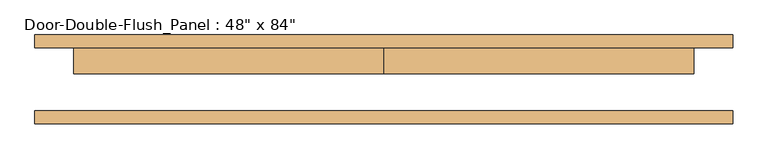
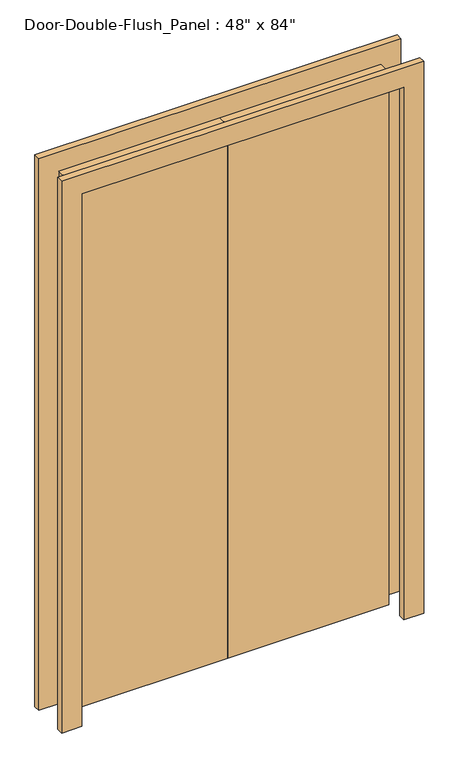
"""IFC4 building model written with IfcOpenShell, lengths in millimetres: door geometry."""

import ifcopenshell
import ifcopenshell.guid

model = None  # the IFC model being written
_history = None  # IfcOwnerHistory: only IFC2X3 demands one
_inside = {}  # id of a spatial element -> (the spatial element, [elements in it])
_under = {}  # id of a project, library or spatial element -> (it, [spatial elements below it])
_declared = {}  # id of a project -> (the project, [libraries it declares])
_typed = {}  # id of a type object -> (the type object, [elements of that type])
_made_of = {}  # id of a material, layer set ... -> (it, [elements and type objects made of it])


def new_model(schema):
    """Start an empty IFC model of exactly this schema.

    Asked for "IFC4X3", IfcOpenShell would pick the latest addendum, in which some entities
    have other attributes; the version numbers below select the first issue.
    IFC2X3 requires an IfcOwnerHistory on every rooted entity: one is made here for all.
    """
    global model, _history
    if schema == "IFC4X3":
        model = ifcopenshell.file(schema_version=(4, 3, 0, 0))
    else:
        model = ifcopenshell.file(schema=schema)
    _inside.clear()
    _under.clear()
    _declared.clear()
    _typed.clear()
    _made_of.clear()
    _history = None
    if model.schema == "IFC2X3":
        org = make("IfcOrganization", Name="unknown")
        user = make(
            "IfcPersonAndOrganization",
            ThePerson=make("IfcPerson", FamilyName="unknown"),
            TheOrganization=org,
        )
        app = make(
            "IfcApplication",
            ApplicationDeveloper=org,
            Version="unknown",
            ApplicationFullName="unknown",
            ApplicationIdentifier="unknown",
        )
        _history = make(
            "IfcOwnerHistory",
            OwningUser=user,
            OwningApplication=app,
            ChangeAction="ADDED",
            CreationDate=0,
        )
    return model


def make(cls, **values):
    """One entity of the class cls with the attributes given. An attribute that is None is left unset."""
    return model.create_entity(
        cls, **{name: value for name, value in values.items() if value is not None}
    )


def rooted(cls, **values):
    """An entity with a GlobalId (a new one), such as an element, a storey or a relation."""
    return make(cls, GlobalId=ifcopenshell.guid.new(), OwnerHistory=_history, **values)


def si_unit(unit_type, name, prefix=None):
    """IfcSIUnit, for example si_unit("LENGTHUNIT", "METRE", prefix="MILLI")."""
    return make("IfcSIUnit", UnitType=unit_type, Prefix=prefix, Name=name)


def assignment(units):
    """IfcUnitAssignment: the units of a project."""
    return None if units is None else make("IfcUnitAssignment", Units=units)


def point(xyz):
    """IfcCartesianPoint."""
    return None if xyz is None else make("IfcCartesianPoint", Coordinates=xyz)


def direction(xyz):
    """IfcDirection."""
    return None if xyz is None else make("IfcDirection", DirectionRatios=xyz)


def frame(location, z_axis=None, x_axis=None):
    """IfcAxis2Placement3D, a coordinate frame: its origin and axes. An axis left out is left unset."""
    return make(
        "IfcAxis2Placement3D",
        Location=point(location),
        Axis=direction(z_axis),
        RefDirection=direction(x_axis),
    )


def origin():
    """The frame at (0, 0, 0) with its axes left unset."""
    return frame((0.0, 0.0, 0.0))


def origin_with_axes():
    """The frame at (0, 0, 0) with the z axis (0, 0, 1) and the x axis (1, 0, 0) written out."""
    return frame((0.0, 0.0, 0.0), z_axis=(0.0, 0.0, 1.0), x_axis=(1.0, 0.0, 0.0))


def place(relative_to, where):
    """IfcLocalPlacement: puts the frame where relative to a parent placement (None: the world)."""
    return make(
        "IfcLocalPlacement", PlacementRelTo=relative_to, RelativePlacement=where
    )


def context(
    kind, dimensions, precision=None, world=None, true_north=None, identifier=None
):
    """IfcGeometricRepresentationContext, for example the 3D "Model" context."""
    return make(
        "IfcGeometricRepresentationContext",
        ContextIdentifier=identifier,
        ContextType=kind,
        CoordinateSpaceDimension=dimensions,
        Precision=precision,
        WorldCoordinateSystem=world,
        TrueNorth=true_north,
    )


def project(units=None, contexts=None):
    """IfcProject with its units and contexts."""
    return rooted(
        "IfcProject",
        Name="project",
        RepresentationContexts=contexts,
        UnitsInContext=assignment(units),
    )


def spatial(cls, under=None, at=None, **own):
    """A site, building, storey or space (cls), placed at a placement, below another one or the project."""
    s = rooted(cls, ObjectPlacement=at, **own)
    if under is not None:
        _under.setdefault(under.id(), (under, []))[1].append(s)
    return s


def polyline(points):
    """IfcPolyline through the points."""
    return make("IfcPolyline", Points=[point(p) for p in points])


def outline(outer, holes=None, kind="AREA"):
    """IfcArbitraryClosedProfileDef: a profile drawn as a closed curve; with holes, ...WithVoids."""
    if holes is None:
        return make("IfcArbitraryClosedProfileDef", ProfileType=kind, OuterCurve=outer)
    return make(
        "IfcArbitraryProfileDefWithVoids",
        ProfileType=kind,
        OuterCurve=outer,
        InnerCurves=holes,
    )


def extrude(swept, where, along, depth):
    """IfcExtrudedAreaSolid: the profile swept, set in the frame where, extruded along a direction by depth."""
    return make(
        "IfcExtrudedAreaSolid",
        SweptArea=swept,
        Position=where,
        ExtrudedDirection=direction(along),
        Depth=depth,
    )


def shape(context_of_items, identifier, shape_type, items):
    """IfcShapeRepresentation: the items that make up one representation, for example the "Body"."""
    return make(
        "IfcShapeRepresentation",
        ContextOfItems=context_of_items,
        RepresentationIdentifier=identifier,
        RepresentationType=shape_type,
        Items=items,
    )


def source(mapping_origin, context_of_items, identifier, shape_type, items):
    """IfcRepresentationMap: a shape defined once, which mapped items show again and again."""
    return make(
        "IfcRepresentationMap",
        MappingOrigin=mapping_origin,
        MappedRepresentation=shape(context_of_items, identifier, shape_type, items),
    )


def transform(
    local_origin,
    x_axis=None,
    y_axis=None,
    z_axis=None,
    scale=None,
    scale2=None,
    scale3=None,
    uniform=True,
):
    """IfcCartesianTransformationOperator3D, or its non-uniform kind. x_axis, y_axis, z_axis: its Axis1, 2, 3."""
    if uniform:
        return make(
            "IfcCartesianTransformationOperator3D",
            Axis1=direction(x_axis),
            Axis2=direction(y_axis),
            LocalOrigin=point(local_origin),
            Scale=scale,
            Axis3=direction(z_axis),
        )
    return make(
        "IfcCartesianTransformationOperator3DnonUniform",
        Axis1=direction(x_axis),
        Axis2=direction(y_axis),
        LocalOrigin=point(local_origin),
        Scale=scale,
        Axis3=direction(z_axis),
        Scale2=scale2,
        Scale3=scale3,
    )


def mapped(mapping_source, mapping_target):
    """IfcMappedItem: shows the shape of a source again, moved by a transform."""
    return make(
        "IfcMappedItem", MappingSource=mapping_source, MappingTarget=mapping_target
    )


def made_of(thing, what):
    """Note that an element or type object is made of a material, layer set ...; save() writes the relation."""
    if what is not None:
        _made_of.setdefault(what.id(), (what, []))[1].append(thing)
    return thing


def element(
    cls,
    number,
    at=None,
    inside=None,
    cuts=None,
    type_object=None,
    material=None,
    context=None,
    identifier="Body",
    shape_type=None,
    held_by="IfcProductDefinitionShape",
    body=None,
    shapes=None,
    **own,
):
    """One element of the class cls, such as IfcWall. Its Tag is "e" and its number.

    at: its placement. inside: the storey or other place that contains it. cuts: it is an
    opening in that element (IfcRelVoidsElement). A single representation is given by context,
    identifier, shape_type and body (its items); several are given by shapes. held_by: the class
    of the entity that holds the representations. save() writes the other relations.
    """
    e = rooted(cls, Tag="e%d" % number, ObjectPlacement=at, **own)
    if body is not None:
        shapes = [shape(context, identifier, shape_type, body)]
    if shapes is not None:
        e.Representation = make(held_by, Representations=shapes)
    if inside is not None:
        _inside.setdefault(inside.id(), (inside, []))[1].append(e)
    if cuts is not None:
        rooted(
            "IfcRelVoidsElement", RelatingBuildingElement=cuts, RelatedOpeningElement=e
        )
    if type_object is not None:
        _typed.setdefault(type_object.id(), (type_object, []))[1].append(e)
    return made_of(e, material)


def aggregate(whole, parts):
    """IfcRelAggregates: a whole, such as a stair, and the parts it consists of."""
    return rooted("IfcRelAggregates", RelatingObject=whole, RelatedObjects=parts)


def save(model, path):
    """Write the relations noted so far, then the file.

    IfcRelAggregates (storeys below a building ...), IfcRelContainedInSpatialStructure (elements
    in a storey), IfcRelDefinesByType, IfcRelAssociatesMaterial and IfcRelDeclares: one each for
    every whole, place, type object, material and project.
    """
    for whole, parts in _under.values():
        aggregate(whole, parts)
    for where, things in _inside.values():
        rooted(
            "IfcRelContainedInSpatialStructure",
            RelatedElements=things,
            RelatingStructure=where,
        )
    for kind, things in _typed.values():
        rooted("IfcRelDefinesByType", RelatedObjects=things, RelatingType=kind)
    for what, things in _made_of.values():
        rooted("IfcRelAssociatesMaterial", RelatedObjects=things, RelatingMaterial=what)
    for by, libraries in _declared.values():
        rooted("IfcRelDeclares", RelatingContext=by, RelatedDefinitions=libraries)
    model.write(path)


def door_4331e645(model_context):
    return source(origin(), model_context, "Body", "SweptSolid", [
        extrude(outline(polyline([(2133.6, -609.6), (2133.6, 609.6), (0.0, 609.6), (0.0, 685.8), (2209.8, 685.8), (2209.8, -685.8), (0.0, -685.8), (0.0, -609.6), (2133.6, -609.6)])), frame((0.0, -87.3125, 0.0), z_axis=(0.0, 1.0, 0.0), x_axis=(0.0, 0.0, 1.0)), (0.0, 0.0, 1.0), 25.4),
        extrude(outline(polyline([(2133.6, -609.6), (2133.6, 609.6), (0.0, 609.6), (0.0, 685.8), (2209.8, 685.8), (2209.8, -685.8), (0.0, -685.8), (0.0, -609.6), (2133.6, -609.6)])), frame((0.0, 61.9125, 0.0), z_axis=(0.0, 1.0, 0.0), x_axis=(0.0, 0.0, 1.0)), (0.0, 0.0, 1.0), 25.4),
        extrude(outline(polyline([(0.0, 61.9125), (609.6, 61.9125), (609.6, 11.1125), (0.0, 11.1125), (0.0, 61.9125)])), origin_with_axes(), (0.0, 0.0, 1.0), 2133.6),
        extrude(outline(polyline([(-609.6, 61.9125), (0.0, 61.9125), (0.0, 11.1125), (-609.6, 11.1125), (-609.6, 61.9125)])), origin_with_axes(), (0.0, 0.0, 1.0), 2133.6),
    ])


if __name__ == "__main__":
    model = new_model("IFC4")
    model_context = context("Model", 3, world=origin())
    ifc_project = project(units=[si_unit("LENGTHUNIT", "METRE", prefix="MILLI")], contexts=[model_context])
    site = spatial("IfcSite", under=ifc_project)
    building = spatial("IfcBuilding", under=site)
    placement = place(None, origin())
    door_shape = door_4331e645(model_context)
    element("IfcDoor", 1, ObjectType="Door-Double-Flush_Panel : 48\" x 84\"", at=placement, inside=building, context=model_context, shape_type="MappedRepresentation", body=[
        mapped(door_shape, transform((0.0, 0.0, 0.0), x_axis=(1.0, 0.0, 0.0), y_axis=(0.0, 1.0, 0.0), z_axis=(0.0, 0.0, 1.0))),
    ])
    save(model, "model.ifc")

# Revit data of these elements
# Type "Door-Double-Flush_Panel : 48\" x 84\""
#   Type Mark = "8"
#   Fire Rating = "60 Mins"
#   Construction Type Id = "DOOR"
#   Assembly Code = "C1020"
#   Analytic Construction = "Wooden"
#   Thickness = 0' - 2"
#   Thermal Resistance (R) = 2.5876 (h·ft²·°F)/BTU
#   Swing Angle [instance default] = 90.00°
#   Panel Width = 2' - 0"
#   Heat Transfer Coefficient (U) = 0.3865 BTU/(h·ft²·°F)
#   Height = 7' - 0"
#   Trim Projection Ext = 0' - 1"
#   Trim Projection Int = 0' - 1"
#   Trim Width = 0' - 3"
#   Width = 4' - 0"
#   Define Thermal Properties by = 1
#   Panel Material = Wood - Birch - Solid Stained Light Low Gloss
#   Trim Material = Paint - Sienna
#   Visual Light Transmittance = 0
#   Solar Heat Gain Coefficient = 0
#   Function = (empty or 0)
#   Wall Closure = (empty or 0)
# Element 1 (IfcDoor, "Door-Double-Flush_Panel : 48\" x 84\"")
#   Materials on its faces: "Paint - Sienna", "Wood - Birch - Solid Stained Light Low Gloss"
# Materials
#   "Wood - Birch - Solid Stained Light Low Gloss": class "Wood", colour RGB 210 159 95, transparency 0, Cost = 0
#   "Paint - Sienna": class "Miscellaneous", colour RGB 118 70 51, transparency 0, Cost = 0
